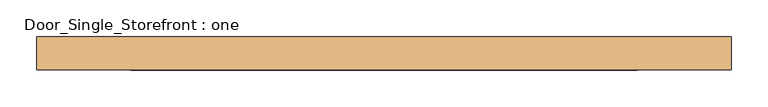
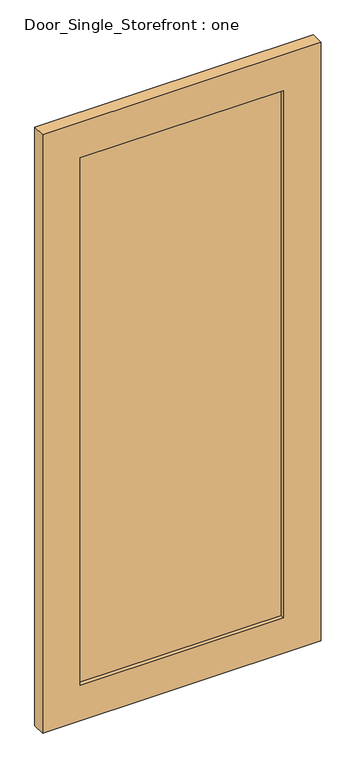
"""IFC4 building model written with IfcOpenShell, lengths in millimetres: door geometry, Door_Single_Storefront : one."""

from ifc_helpers import new_model, si_unit, frame, origin, place, context, project, spatial, polyline, outline, extrude, source, transform, mapped, element, save


def door_single_storefront_one_e7c4c47f(model_context):
    return source(origin(), model_context, "Body", "SweptSolid", [
        extrude(outline(polyline([(342.9, -6.35), (-342.9, -6.35), (-342.9, 12.7), (342.9, 12.7), (342.9, -6.35)])), frame((0.0, 0.0, 127.0), z_axis=(0.0, 0.0, 1.0), x_axis=(1.0, 0.0, 0.0)), (0.0, 0.0, 1.0), 1879.6),
        extrude(outline(polyline([(2133.6, -469.9), (0.0, -469.9), (0.0, 469.9), (2133.6, 469.9), (2133.6, -469.9)]), holes=[polyline([(127.0, 342.9), (127.0, -342.9), (2006.6, -342.9), (2006.6, 342.9), (127.0, 342.9)])]), frame((0.0, -19.05, 0.0), z_axis=(0.0, 1.0, 0.0), x_axis=(0.0, 0.0, 1.0)), (0.0, 0.0, 1.0), 44.45),
    ])


if __name__ == "__main__":
    model = new_model("IFC4")
    model_context = context("Model", 3, world=origin())
    ifc_project = project(units=[si_unit("LENGTHUNIT", "METRE", prefix="MILLI")], contexts=[model_context])
    site = spatial("IfcSite", under=ifc_project)
    building = spatial("IfcBuilding", under=site)
    placement = place(None, origin())
    door_single_storefront_one_shape = door_single_storefront_one_e7c4c47f(model_context)
    element("IfcDoor", 1, ObjectType="Door_Single_Storefront : one", at=placement, inside=building, context=model_context, shape_type="MappedRepresentation", body=[
        mapped(door_single_storefront_one_shape, transform((0.0, 0.0, 0.0), x_axis=(1.0, 0.0, 0.0), y_axis=(0.0, 1.0, 0.0), z_axis=(0.0, 0.0, 1.0))),
    ])
    save(model, "model.ifc")

# Revit data of these elements
# Type "Door_Single_Storefront : one"
#   Type Mark = "22"
#   Analytic Construction = "<None>"
#   Stile_Width = 0' - 5"
#   Door_Thickness = 0' - 1 3/4"
#   Door_Offset = 0' - 1"
#   Glass_Material = Glass
#   Frame_Material = Door - Panel
#   Function = (empty or 0)
# Element 1 (IfcDoor, "Door_Single_Storefront : one")
#   Materials on its faces: "Door - Panel", "Glass"
# Materials
#   "Glass": class "Glass", colour RGB 218 227 224, transparency 0.85, Description = "Soda Lime Glass", Cost = 0
#   "Door - Panel": class "Wood", colour RGB 114 82 51, transparency 0
